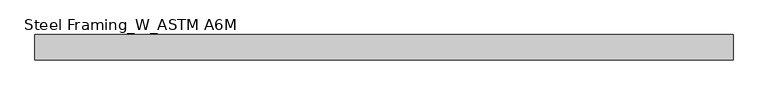
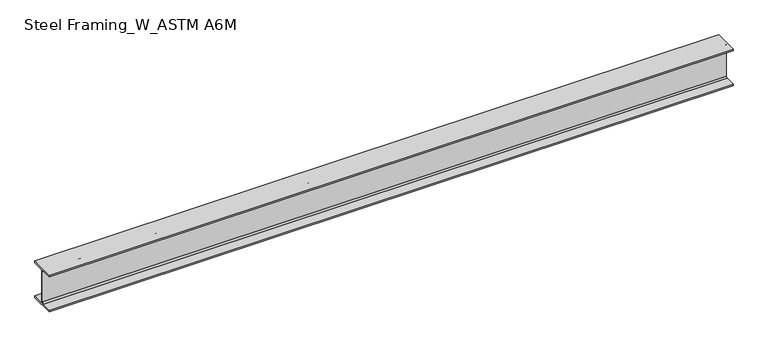
"""IFC4 building model written with IfcOpenShell, lengths in millimetres: beam geometry, Steel Framing_W_ASTM A6M : H_SB_AR_S02_W200x31.3_B6."""

import ifcopenshell
import ifcopenshell.guid

model = None  # the IFC model being written
_history = None  # IfcOwnerHistory: only IFC2X3 demands one
_inside = {}  # id of a spatial element -> (the spatial element, [elements in it])
_under = {}  # id of a project, library or spatial element -> (it, [spatial elements below it])
_declared = {}  # id of a project -> (the project, [libraries it declares])
_typed = {}  # id of a type object -> (the type object, [elements of that type])
_made_of = {}  # id of a material, layer set ... -> (it, [elements and type objects made of it])


def new_model(schema):
    """Start an empty IFC model of exactly this schema.

    Asked for "IFC4X3", IfcOpenShell would pick the latest addendum, in which some entities
    have other attributes; the version numbers below select the first issue.
    IFC2X3 requires an IfcOwnerHistory on every rooted entity: one is made here for all.
    """
    global model, _history
    if schema == "IFC4X3":
        model = ifcopenshell.file(schema_version=(4, 3, 0, 0))
    else:
        model = ifcopenshell.file(schema=schema)
    _inside.clear()
    _under.clear()
    _declared.clear()
    _typed.clear()
    _made_of.clear()
    _history = None
    if model.schema == "IFC2X3":
        org = make("IfcOrganization", Name="unknown")
        user = make(
            "IfcPersonAndOrganization",
            ThePerson=make("IfcPerson", FamilyName="unknown"),
            TheOrganization=org,
        )
        app = make(
            "IfcApplication",
            ApplicationDeveloper=org,
            Version="unknown",
            ApplicationFullName="unknown",
            ApplicationIdentifier="unknown",
        )
        _history = make(
            "IfcOwnerHistory",
            OwningUser=user,
            OwningApplication=app,
            ChangeAction="ADDED",
            CreationDate=0,
        )
    return model


def make(cls, **values):
    """One entity of the class cls with the attributes given. An attribute that is None is left unset."""
    return model.create_entity(
        cls, **{name: value for name, value in values.items() if value is not None}
    )


def rooted(cls, **values):
    """An entity with a GlobalId (a new one), such as an element, a storey or a relation."""
    return make(cls, GlobalId=ifcopenshell.guid.new(), OwnerHistory=_history, **values)


def si_unit(unit_type, name, prefix=None):
    """IfcSIUnit, for example si_unit("LENGTHUNIT", "METRE", prefix="MILLI")."""
    return make("IfcSIUnit", UnitType=unit_type, Prefix=prefix, Name=name)


def assignment(units):
    """IfcUnitAssignment: the units of a project."""
    return None if units is None else make("IfcUnitAssignment", Units=units)


def point(xyz):
    """IfcCartesianPoint."""
    return None if xyz is None else make("IfcCartesianPoint", Coordinates=xyz)


def direction(xyz):
    """IfcDirection."""
    return None if xyz is None else make("IfcDirection", DirectionRatios=xyz)


def frame(location, z_axis=None, x_axis=None):
    """IfcAxis2Placement3D, a coordinate frame: its origin and axes. An axis left out is left unset."""
    return make(
        "IfcAxis2Placement3D",
        Location=point(location),
        Axis=direction(z_axis),
        RefDirection=direction(x_axis),
    )


def frame_2d(location, x_axis=None):
    """IfcAxis2Placement2D, a coordinate frame in the plane: its origin and x axis."""
    return make(
        "IfcAxis2Placement2D", Location=point(location), RefDirection=direction(x_axis)
    )


def origin():
    """The frame at (0, 0, 0) with its axes left unset."""
    return frame((0.0, 0.0, 0.0))


def place(relative_to, where):
    """IfcLocalPlacement: puts the frame where relative to a parent placement (None: the world)."""
    return make(
        "IfcLocalPlacement", PlacementRelTo=relative_to, RelativePlacement=where
    )


def context(
    kind, dimensions, precision=None, world=None, true_north=None, identifier=None
):
    """IfcGeometricRepresentationContext, for example the 3D "Model" context."""
    return make(
        "IfcGeometricRepresentationContext",
        ContextIdentifier=identifier,
        ContextType=kind,
        CoordinateSpaceDimension=dimensions,
        Precision=precision,
        WorldCoordinateSystem=world,
        TrueNorth=true_north,
    )


def project(units=None, contexts=None):
    """IfcProject with its units and contexts."""
    return rooted(
        "IfcProject",
        Name="project",
        RepresentationContexts=contexts,
        UnitsInContext=assignment(units),
    )


def spatial(cls, under=None, at=None, **own):
    """A site, building, storey or space (cls), placed at a placement, below another one or the project."""
    s = rooted(cls, ObjectPlacement=at, **own)
    if under is not None:
        _under.setdefault(under.id(), (under, []))[1].append(s)
    return s


def polyline(points):
    """IfcPolyline through the points."""
    return make("IfcPolyline", Points=[point(p) for p in points])


def circle_curve(where, radius):
    """IfcCircle in the frame where."""
    return make("IfcCircle", Position=where, Radius=radius)


def trimmed(basis, trim1, trim2, sense, master):
    """IfcTrimmedCurve: the piece of a basis curve between two trims."""
    return make(
        "IfcTrimmedCurve",
        BasisCurve=basis,
        Trim1=trim1,
        Trim2=trim2,
        SenseAgreement=sense,
        MasterRepresentation=master,
    )


def segment(curve, same_sense, transition):
    """IfcCompositeCurveSegment."""
    return make(
        "IfcCompositeCurveSegment",
        Transition=transition,
        SameSense=same_sense,
        ParentCurve=curve,
    )


def composite_curve(segments, self_intersect=None):
    """IfcCompositeCurve: segments joined end to end."""
    return make("IfcCompositeCurve", Segments=segments, SelfIntersect=self_intersect)


def outline(outer, holes=None, kind="AREA"):
    """IfcArbitraryClosedProfileDef: a profile drawn as a closed curve; with holes, ...WithVoids."""
    if holes is None:
        return make("IfcArbitraryClosedProfileDef", ProfileType=kind, OuterCurve=outer)
    return make(
        "IfcArbitraryProfileDefWithVoids",
        ProfileType=kind,
        OuterCurve=outer,
        InnerCurves=holes,
    )


def extrude(swept, where, along, depth):
    """IfcExtrudedAreaSolid: the profile swept, set in the frame where, extruded along a direction by depth."""
    return make(
        "IfcExtrudedAreaSolid",
        SweptArea=swept,
        Position=where,
        ExtrudedDirection=direction(along),
        Depth=depth,
    )


def shape(context_of_items, identifier, shape_type, items):
    """IfcShapeRepresentation: the items that make up one representation, for example the "Body"."""
    return make(
        "IfcShapeRepresentation",
        ContextOfItems=context_of_items,
        RepresentationIdentifier=identifier,
        RepresentationType=shape_type,
        Items=items,
    )


def source(mapping_origin, context_of_items, identifier, shape_type, items):
    """IfcRepresentationMap: a shape defined once, which mapped items show again and again."""
    return make(
        "IfcRepresentationMap",
        MappingOrigin=mapping_origin,
        MappedRepresentation=shape(context_of_items, identifier, shape_type, items),
    )


def transform(
    local_origin,
    x_axis=None,
    y_axis=None,
    z_axis=None,
    scale=None,
    scale2=None,
    scale3=None,
    uniform=True,
):
    """IfcCartesianTransformationOperator3D, or its non-uniform kind. x_axis, y_axis, z_axis: its Axis1, 2, 3."""
    if uniform:
        return make(
            "IfcCartesianTransformationOperator3D",
            Axis1=direction(x_axis),
            Axis2=direction(y_axis),
            LocalOrigin=point(local_origin),
            Scale=scale,
            Axis3=direction(z_axis),
        )
    return make(
        "IfcCartesianTransformationOperator3DnonUniform",
        Axis1=direction(x_axis),
        Axis2=direction(y_axis),
        LocalOrigin=point(local_origin),
        Scale=scale,
        Axis3=direction(z_axis),
        Scale2=scale2,
        Scale3=scale3,
    )


def mapped(mapping_source, mapping_target):
    """IfcMappedItem: shows the shape of a source again, moved by a transform."""
    return make(
        "IfcMappedItem", MappingSource=mapping_source, MappingTarget=mapping_target
    )


def made_of(thing, what):
    """Note that an element or type object is made of a material, layer set ...; save() writes the relation."""
    if what is not None:
        _made_of.setdefault(what.id(), (what, []))[1].append(thing)
    return thing


def element(
    cls,
    number,
    at=None,
    inside=None,
    cuts=None,
    type_object=None,
    material=None,
    context=None,
    identifier="Body",
    shape_type=None,
    held_by="IfcProductDefinitionShape",
    body=None,
    shapes=None,
    **own,
):
    """One element of the class cls, such as IfcWall. Its Tag is "e" and its number.

    at: its placement. inside: the storey or other place that contains it. cuts: it is an
    opening in that element (IfcRelVoidsElement). A single representation is given by context,
    identifier, shape_type and body (its items); several are given by shapes. held_by: the class
    of the entity that holds the representations. save() writes the other relations.
    """
    e = rooted(cls, Tag="e%d" % number, ObjectPlacement=at, **own)
    if body is not None:
        shapes = [shape(context, identifier, shape_type, body)]
    if shapes is not None:
        e.Representation = make(held_by, Representations=shapes)
    if inside is not None:
        _inside.setdefault(inside.id(), (inside, []))[1].append(e)
    if cuts is not None:
        rooted(
            "IfcRelVoidsElement", RelatingBuildingElement=cuts, RelatedOpeningElement=e
        )
    if type_object is not None:
        _typed.setdefault(type_object.id(), (type_object, []))[1].append(e)
    return made_of(e, material)


def aggregate(whole, parts):
    """IfcRelAggregates: a whole, such as a stair, and the parts it consists of."""
    return rooted("IfcRelAggregates", RelatingObject=whole, RelatedObjects=parts)


def save(model, path):
    """Write the relations noted so far, then the file.

    IfcRelAggregates (storeys below a building ...), IfcRelContainedInSpatialStructure (elements
    in a storey), IfcRelDefinesByType, IfcRelAssociatesMaterial and IfcRelDeclares: one each for
    every whole, place, type object, material and project.
    """
    for whole, parts in _under.values():
        aggregate(whole, parts)
    for where, things in _inside.values():
        rooted(
            "IfcRelContainedInSpatialStructure",
            RelatedElements=things,
            RelatingStructure=where,
        )
    for kind, things in _typed.values():
        rooted("IfcRelDefinesByType", RelatedObjects=things, RelatingType=kind)
    for what, things in _made_of.values():
        rooted("IfcRelAssociatesMaterial", RelatedObjects=things, RelatingMaterial=what)
    for by, libraries in _declared.values():
        rooted("IfcRelDeclares", RelatingContext=by, RelatedDefinitions=libraries)
    model.write(path)


def steel_framing_w_astm_a6m_5d0dfb1e(model_context):
    return source(origin(), model_context, "Body", "SweptSolid", [
        extrude(outline(composite_curve([segment(polyline([(67.0, -94.8), (67.0, -105.0), (-67.0, -105.0), (-67.0, -94.8), (-10.775, -94.8)]), True, "CONTINUOUS"), segment(trimmed(circle_curve(frame_2d((-10.775, -87.2)), 7.6), [point((-10.775, -94.8))], [point((-3.175, -87.2))], True, "CARTESIAN"), True, "CONTINUOUS"), segment(polyline([(-3.175, -87.2), (-3.175, 87.2)]), True, "CONTINUOUS"), segment(trimmed(circle_curve(frame_2d((-10.775, 87.2)), 7.6), [point((-3.175, 87.2))], [point((-10.775, 94.8))], True, "CARTESIAN"), True, "CONTINUOUS"), segment(polyline([(-10.775, 94.8), (-67.0, 94.8), (-67.0, 105.0), (67.0, 105.0), (67.0, 94.8), (10.775, 94.8)]), True, "CONTINUOUS"), segment(trimmed(circle_curve(frame_2d((10.775, 87.2)), 7.6), [point((10.775, 94.8))], [point((3.175, 87.2))], True, "CARTESIAN"), True, "CONTINUOUS"), segment(polyline([(3.175, 87.2), (3.175, -87.2)]), True, "CONTINUOUS"), segment(trimmed(circle_curve(frame_2d((10.775, -87.2)), 7.6), [point((3.175, -87.2))], [point((10.775, -94.8))], True, "CARTESIAN"), True, "CONTINUOUS"), segment(polyline([(10.775, -94.8), (67.0, -94.8)]), True, "CONTINUOUS")], self_intersect=False)), frame((-1846.3, 0.0, 0.0), z_axis=(1.0, 0.0, 0.0), x_axis=(0.0, 1.0, 0.0)), (0.0, 0.0, 1.0), 3692.6),
    ])


if __name__ == "__main__":
    model = new_model("IFC4")
    model_context = context("Model", 3, world=origin())
    ifc_project = project(units=[si_unit("LENGTHUNIT", "METRE", prefix="MILLI")], contexts=[model_context])
    site = spatial("IfcSite", under=ifc_project)
    building = spatial("IfcBuilding", under=site)
    placement = place(None, origin())
    steel_framing_w_astm_a6m_shape = steel_framing_w_astm_a6m_5d0dfb1e(model_context)
    element("IfcBeam", 1, ObjectType="Steel Framing_W_ASTM A6M : H_SB_AR_S02_W200x31.3_B6", at=placement, inside=building, context=model_context, shape_type="MappedRepresentation", body=[
        mapped(steel_framing_w_astm_a6m_shape, transform((0.0, 0.0, 0.0), x_axis=(1.0, 0.0, 0.0), y_axis=(0.0, 1.0, 0.0), z_axis=(0.0, 0.0, 1.0))),
    ])
    save(model, "model.ifc")

# Revit data of these elements
# Type "Steel Framing_W_ASTM A6M : H_SB_AR_S02_W200x31.3_B6"
#   Type Mark = "B6"
#   Section Name Key = "W8x21"
#   Width = 13.4 cm
#   Web Thickness = 0.635 cm
#   Web Fillet = 0.76 cm
#   Warping Constant = 40800.0 cm⁶
#   Torsional Moment of Inertia = 11.70 cm⁴
#   Section Area = 39.7 cm²
#   Plastic Modulus weak axis = 93.2 cm³
#   Plastic Modulus strong axis = 334.0 cm³
#   Perimeter = 0.93 m²/m
#   Nominal Weight = 31.30 kgf/m
#   Moment of Inertia weak axis = 407.00 cm⁴
#   Moment of Inertia strong axis = 3130.00 cm⁴
#   Height = 21.0 cm
#   Flange Thickness = 1.02 cm
#   Elastic Modulus weak axis = 60.8 cm³
#   Elastic Modulus strong axis = 298.0 cm³
#   Centroid Vertical = 10.5 cm
#   Centroid Horizontal = 6.7 cm
#   Length [instance default] = 1500 mm
#   Structural Material [instance default] = Steel, 45-345
#   Bolt Spacing = 0
#   Assembly Code = ""
# Element 1 (IfcBeam, "Steel Framing_W_ASTM A6M : H_SB_AR_S02_W200x31.3_B6")
#   Materials on its faces: "Steel, 45-345"
# Materials
#   "Steel, 45-345": class "Metal", colour RGB 189 187 185, transparency 0, Description = "Steel 345 MPa", Cost = 0
